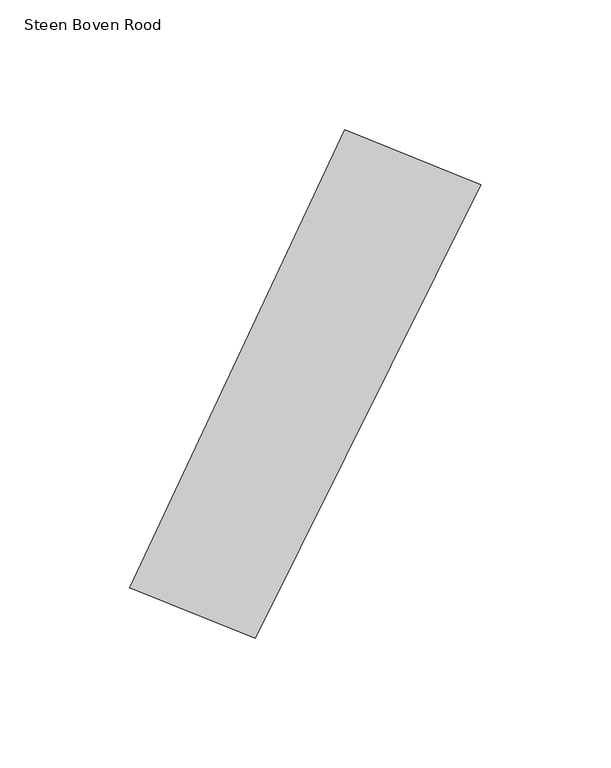
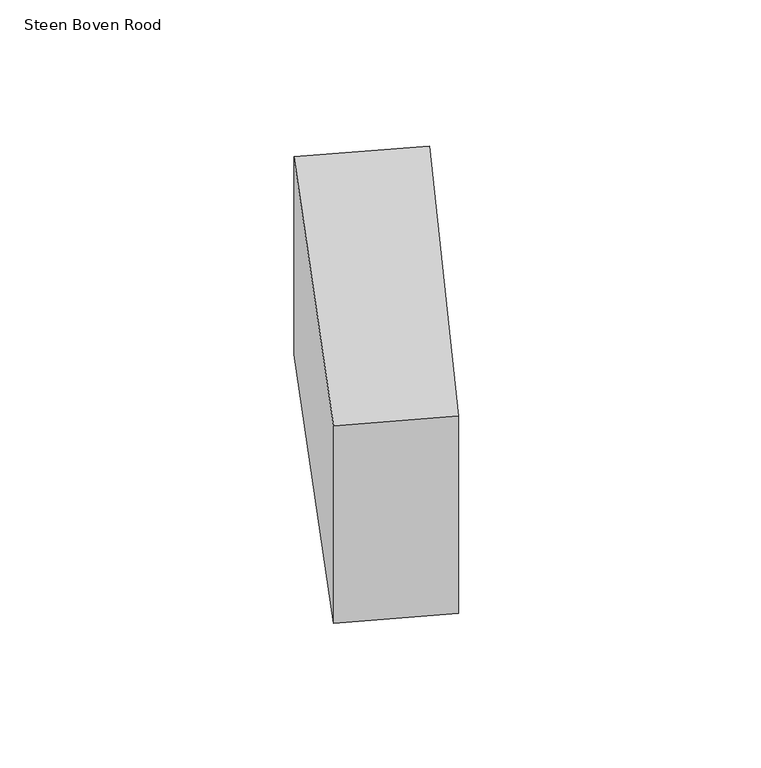
"""IFC4 building model written with IfcOpenShell, lengths in millimetres: proxy geometry, 00_GMA_steen_versie_4 : Steen Boven Rood."""

from ifc_helpers import new_model, si_unit, origin, origin_with_axes, place, context, project, spatial, polyline, outline, extrude, source, transform, mapped, element, save


def steen_boven_rood_52d9d6ee(model_context):
    return source(origin(), model_context, "Body", "SweptSolid", [
        extrude(outline(polyline([(145.5719603, 160.2816805), (58.4880068, -14.8670846), (9.96468, 4.7335986), (93.0275279, 181.4994499), (145.5719603, 160.2816805)])), origin_with_axes(), (0.0, 0.0, 1.0), 100.0),
    ])


if __name__ == "__main__":
    model = new_model("IFC4")
    model_context = context("Model", 3, world=origin())
    ifc_project = project(units=[si_unit("LENGTHUNIT", "METRE", prefix="MILLI")], contexts=[model_context])
    site = spatial("IfcSite", under=ifc_project)
    building = spatial("IfcBuilding", under=site)
    placement = place(None, origin())
    steen_boven_rood_shape = steen_boven_rood_52d9d6ee(model_context)
    element("IfcBuildingElementProxy", 1, Name="00_GMA_steen_versie_4 : Steen Boven Rood", ObjectType="00_GMA_steen_versie_4 : Steen Boven Rood", at=placement, inside=building, context=model_context, shape_type="MappedRepresentation", body=[
        mapped(steen_boven_rood_shape, transform((0.0, 0.0, 0.0), x_axis=(1.0, 0.0, 0.0), y_axis=(0.0, 1.0, 0.0), z_axis=(0.0, 0.0, 1.0))),
    ])
    save(model, "model.ifc")

# Revit data of these elements
# Type "00_GMA_steen_versie_4 : Steen Boven Rood"
#   StootVoegHalfBoven [instance default] = 5 mm
#   StootVoegHalf [instance default] = 5 mm
#   StootVoegBreedteOnder = 10 mm
#   StootVoegBreedteBoven = 10 mm
#   Steendikte = 100 mm
#   LintVoegOnderHalf = 5 mm
#   LintVoegOnder = 10 mm
#   LintVoegBovenHalf = 0 mm
#   LintVoegBoven = 0 mm
#   materiaal = 21_steen_rood
#   MateriaalVoeg = none
#   Default Elevation = 0
# Element 1 (IfcBuildingElementProxy, "00_GMA_steen_versie_4 : Steen Boven Rood")
#   Materials on its faces: "21_steen_rood"
# Materials
#   "21_steen_rood": class "Unassigned", colour RGB 213 111 43, transparency 0, Cost = 0
